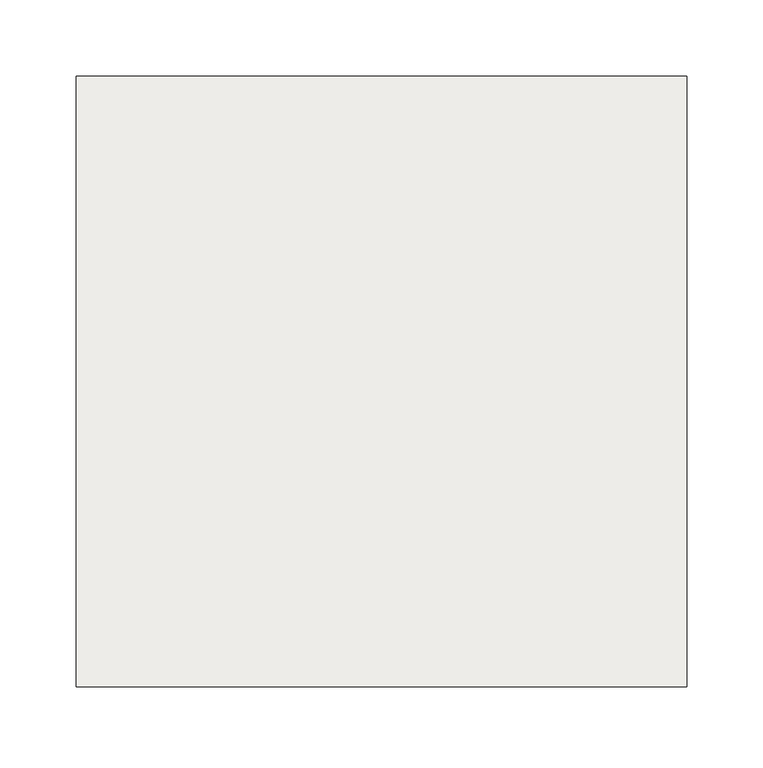
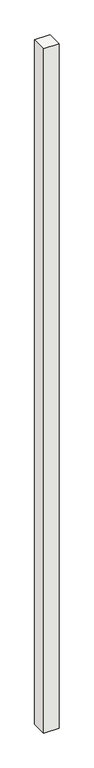
"""IFC4 building model written with IfcOpenShell, lengths in millimetres: footing geometry, NLRS_17_SFO_TLB_funderingspaal geheid beton prefab-AV-MMBPC_gen_rsf : heipaal beton prefab_gen__bxh 400x400."""

from ifc_helpers import new_model, si_unit, frame, origin, place, context, project, spatial, polyline, outline, extrude, source, transform, mapped, element, save


def footing_c87ae41e(model_context):
    return source(origin(), model_context, "Body", "SweptSolid", [
        extrude(outline(polyline([(200.0, -200.0), (-200.0, -200.0), (-200.0, 200.0), (200.0, 200.0), (200.0, -200.0)])), frame((0.0, 0.0, -20000.0), z_axis=(0.0, 0.0, 1.0), x_axis=(1.0, 0.0, 0.0)), (0.0, 0.0, 1.0), 18830.0),
    ])


if __name__ == "__main__":
    model = new_model("IFC4")
    model_context = context("Model", 3, world=origin())
    ifc_project = project(units=[si_unit("LENGTHUNIT", "METRE", prefix="MILLI")], contexts=[model_context])
    site = spatial("IfcSite", under=ifc_project)
    building = spatial("IfcBuilding", under=site)
    placement = place(None, origin())
    footing_shape = footing_c87ae41e(model_context)
    element("IfcFooting", 1, ObjectType="NLRS_17_SFO_TLB_funderingspaal geheid beton prefab-AV-MMBPC_gen_rsf : heipaal beton prefab_gen__bxh 400x400", at=placement, inside=building, context=model_context, shape_type="MappedRepresentation", body=[
        mapped(footing_shape, transform((0.0, 0.0, 0.0), x_axis=(1.0, 0.0, 0.0), y_axis=(0.0, 1.0, 0.0), z_axis=(0.0, 0.0, 1.0))),
    ])
    save(model, "model.ifc")

# Revit data of these elements
# Type "NLRS_17_SFO_TLB_funderingspaal geheid beton prefab-AV-MMBPC_gen_rsf : heipaal beton prefab_gen__bxh 400x400"
#   IfcExportAs = "IfcPile"
#   Type Comments = "prefab heipaal 400x400"
#   Model = " "
#   Manufacturer = " "
#   Description = "prefab heipaal 400x400"
#   Assembly Code = "17.21"
#   Width = 400 mm
#   Slanted Angle [instance default] = 0.00°
#   NLRS_S_draagvermogen_trek [instance default] = 0.00 kN
#   NLRS_S_draagvermogen_druk [instance default] = 0.00 kN
#   NLRS_C_lengte [instance default] = 1660 mm
#   NLRS_C_hoogte = 400 mm
#   NLRS_C_breedte = 400 mm
#   Height [instance default] = 1660 mm
#   Length [instance default] = 1660 mm
#   Angle [instance default] = 0.00°
#   Slanted [instance default] = 0
#   Structural Material = NLRS_f2_beton prefab_gen_rsf
#   Keynote = ""
# Element 1 (IfcFooting, "NLRS_17_SFO_TLB_funderingspaal geheid beton prefab-AV-MMBPC_gen_rsf : heipaal beton prefab_gen__bxh 400x400")
#   NLRS_C_lengte = 18830 mm
#   Height = 18830 mm
#   Length = 18830 mm
#   Materials on its faces: "NLRS_f2_beton prefab_gen_rsf"
# Materials
#   "NLRS_f2_beton prefab_gen_rsf": class "F - Niet gebakken kunststeen", colour RGB 129 133 118, transparency 0, Keynote = "f2", Manufacturer = "Revit Standards Foundation", URL = "www.revitstandards.org", Description = "beton prefab", Cost = 0
